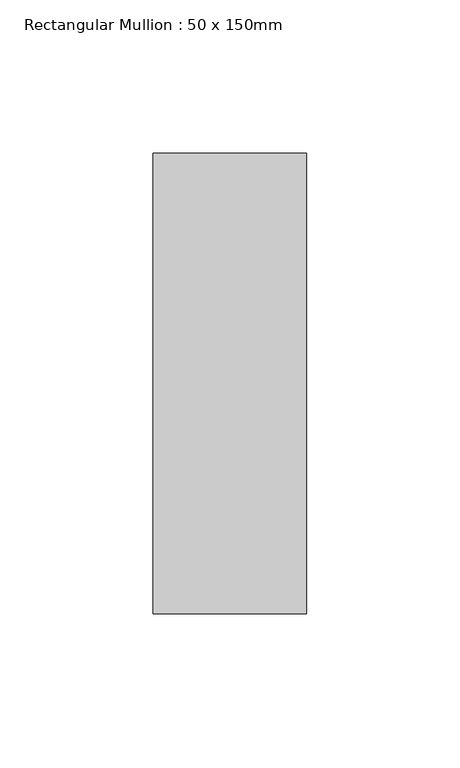
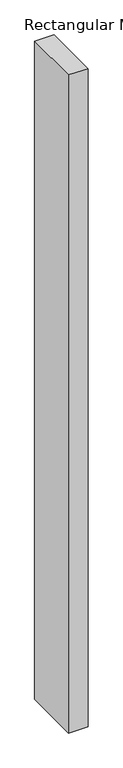
"""IFC4 building model written with IfcOpenShell, lengths in millimetres: member geometry, Rectangular Mullion : 50 x 150mm."""

from ifc_helpers import new_model, si_unit, frame, origin, place, context, project, spatial, polyline, outline, extrude, source, transform, mapped, element, save


def rectangular_mullion_50_x_150mm_b2364271(model_context):
    return source(origin(), model_context, "Body", "SweptSolid", [
        extrude(outline(polyline([(0.0, 75.0), (0.0, -75.0), (-50.0, -75.0), (-50.0, 75.0), (0.0, 75.0)])), frame((0.0, 0.0, -1782.0), z_axis=(0.0, 0.0, 1.0), x_axis=(1.0, 0.0, 0.0)), (0.0, 0.0, 1.0), 1782.0),
    ])


if __name__ == "__main__":
    model = new_model("IFC4")
    model_context = context("Model", 3, world=origin())
    ifc_project = project(units=[si_unit("LENGTHUNIT", "METRE", prefix="MILLI")], contexts=[model_context])
    site = spatial("IfcSite", under=ifc_project)
    building = spatial("IfcBuilding", under=site)
    placement = place(None, origin())
    rectangular_mullion_50_x_150mm_shape = rectangular_mullion_50_x_150mm_b2364271(model_context)
    element("IfcMember", 1, ObjectType="Rectangular Mullion : 50 x 150mm", at=placement, inside=building, context=model_context, shape_type="MappedRepresentation", body=[
        mapped(rectangular_mullion_50_x_150mm_shape, transform((0.0, 0.0, 0.0), x_axis=(1.0, 0.0, 0.0), y_axis=(0.0, 1.0, 0.0), z_axis=(0.0, 0.0, 1.0))),
    ])
    save(model, "model.ifc")

# Revit data of these elements
# Type "Rectangular Mullion : 50 x 150mm"
#   Keynote = "H11"
#   built-in parameter 1007304 = 0.492126 (stored number, unit not read)
#   built-in parameter 1007301 = 0.082021 (stored number, unit not read)
#   built-in parameter 1007300 = 0.082021 (stored number, unit not read)
# Element 1 (IfcMember, "Rectangular Mullion : 50 x 150mm")
#   Materials on its faces: "Aluminium"
# Materials
#   "Aluminium": class "Metal", colour RGB 247 247 247, transparency 0, Description = "Aluminium 6061", Cost = 0
